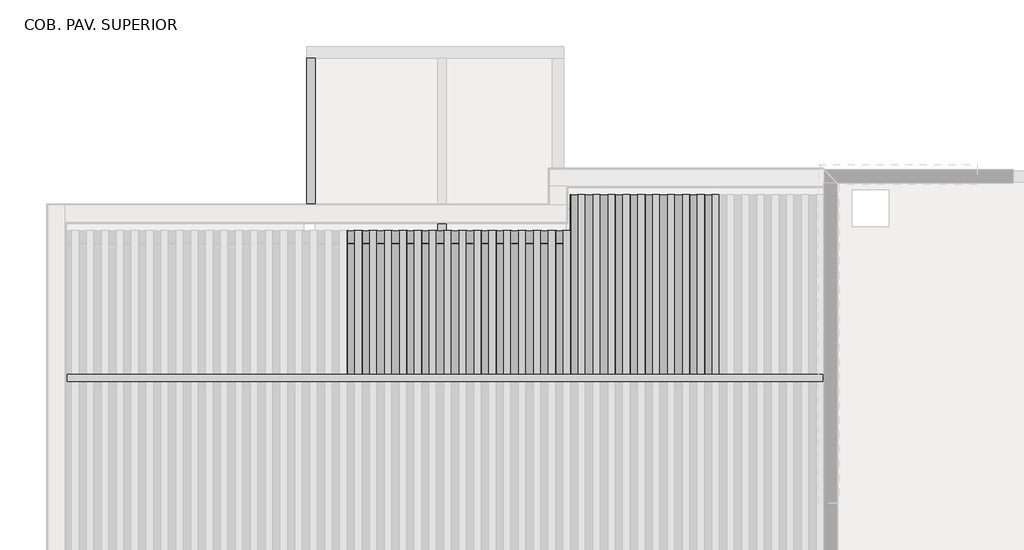
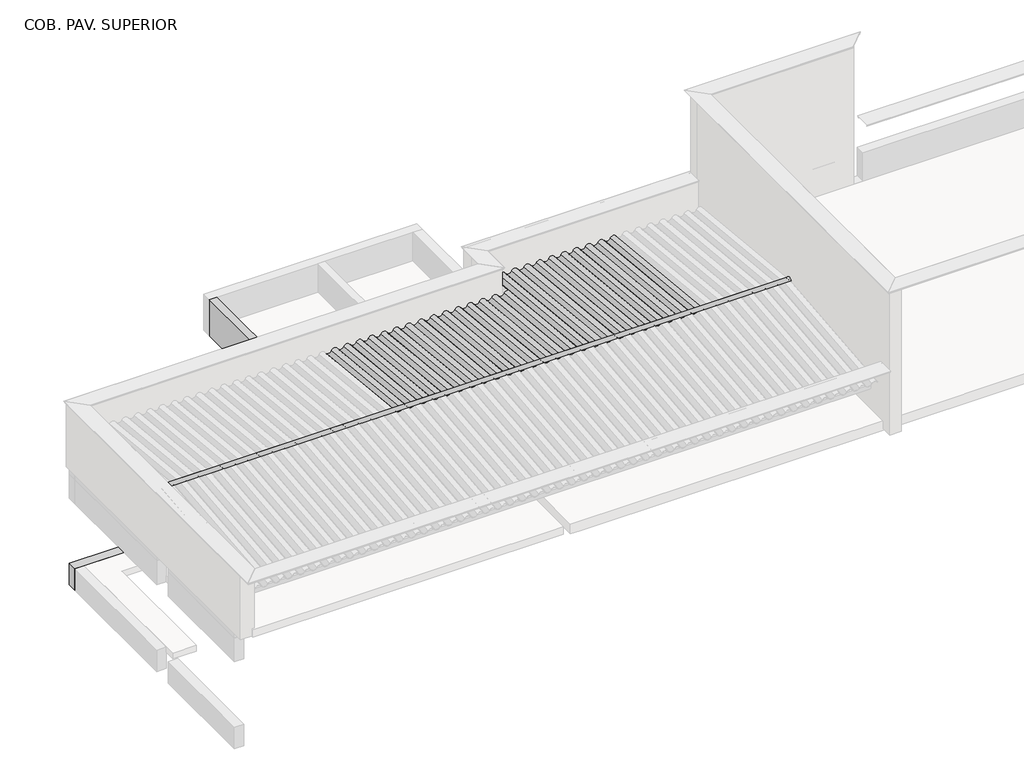
# One storey, part 4 of 7: 41 beams, 9 columns.
# Revit data of these elements (continued)
# Type "Madeira de lei : Berço 6x12cm"
#   A = 0.02 m²
#   Length [instance default] = 1.524 m
#   b = 0.06 m
#   d = 0.12 m
#   Structural Material [instance default] = none
#   Assembly Code = ""
# Type "Cumeeira Telha Ondulada : Fibrocimento"
#   Cost = 5
#   Length [instance default] = 1.524 m
#   b = 0.07 m
#   h = 0.16 m
#   Structural Material = .TELHA DE FIBROCIMENTO
#   Assembly Code = ""
# Type "TQS - Viga retangular : 14.0 x 76.0"
#   Length [instance default] = 1.524 m
#   b = 0.14 m
#   h = 0.76 m
#   Structural Material [instance default] = none
#   Assembly Code = ""
# Type "TQS - Viga retangular : 19.0 x 45.0"
#   Length [instance default] = 1.524 m
#   b = 0.19 m
#   h = 0.45 m
#   Structural Material [instance default] = none
#   Assembly Code = ""
# Type "TQS - Viga retangular : 19.0 x 96.0"
#   Length [instance default] = 1.524 m
#   b = 0.19 m
#   h = 0.96 m
#   Structural Material [instance default] = none
#   Assembly Code = ""
# Type "Telha Ondulada : Fibrocimento"
#   Description = "TELHA ONDULADA FIBROCIMENTO"
#   Cost = 5
#   Length [instance default] = 1.524 m
#   b = 0.07 m
#   h = 0.16 m
#   Structural Material = .TELHA DE FIBROCIMENTO
#   Assembly Code = ""
# Type "Madeira de lei : Viga Cumeeira 6x16cm"
#   A = 0.02 m²
#   Length [instance default] = 1.524 m
#   b = 0.06 m
#   d = 0.16 m
#   Structural Material [instance default] = none
#   Assembly Code = ""
# Type "Madeira de lei-Coluna : Pontalete 6X16cm"
#   A = 0.01952 m²
#   b = 0.06 m
#   d = 0.16 m
#   Structural Material [instance default] = none
#   Assembly Code = ""
# Elements 1, 2, 3, 4, 5, 6, 7, 8, 9 (IfcBeam, "Madeira de lei : Berço 6x12cm")
#   Comments = ""
#   Structural Material = .MADEIRAMENTO
#   Phase Created = CC_PE
#   Materials on its faces: ".MADEIRAMENTO"
# Element 10 (IfcBeam, "Cumeeira Telha Ondulada : Fibrocimento")
#   Comments = ""
#   Phase Created = CC_PE
#   Materials on its faces: ".TELHA DE FIBROCIMENTO"
# Element 11 (IfcBeam, "TQS - Viga retangular : 14.0 x 76.0")
#   Uso = "ESTRUTURA"
#   Titulo = "V415"
#   Chave = "-398"
#   Tipo Elemento = "Viga"
#   SHA1 = "2AA376B6A26CF9712D89C0E8D11BC49B460EBC49"
#   Revisão = ""
#   Tipo de carga = ""
#   Divisor de flexao = ""
#   Secao = ""
#   Configuracao = ""
#   Angulo (graus) = ""
#   Detalhamento = ""
#   Casos de vento manual = ""
#   Tipo = ""
#   Alcas = ""
#   Furos = ""
#   Pino = ""
#   Distribuicao = ""
#   Solidarizado = ""
#   Solidarizar na montagem = ""
#   Unir com o próximo = ""
#   Grupo pre moldado = ""
#   Verificado = ""
#   Concreto C = ""
#   Taxa de armadura (kgf/m³) = 0
#   Carga (tf/m²) = 0
#   Carga (tf/m) = 0
#   Carga (tf) = 0
#   Altura = 0.76 m
#   Rebaixo = -0.40 m
#   Largura = 0.14 m
#   Distancia a face = 0.00 m
#   Distancia ao eixo = 0.00 m
#   Altura gerber esquerda = 0.00 m
#   Largura gerber esquerda = 0.00 m
#   Altura gerber direita = 0.00 m
#   Largura gerber direita = 0.00 m
#   Resultado de Ensaios fck (MPa) = 0
#   Unique TQS ID = -398
#   Principal = yes
#   Structural Material = none
#   Phase Created = CC_PE
# Element 12 (IfcBeam, "TQS - Viga retangular : 14.0 x 76.0")
#   Uso = "ESTRUTURA"
#   Titulo = "V417"
#   Chave = "-400"
#   Tipo Elemento = "Viga"
#   SHA1 = "12908E79E151D5AD934E49BC800BD2D4B155789F"
#   Revisão = ""
#   Tipo de carga = ""
#   Divisor de flexao = ""
#   Secao = ""
#   Configuracao = ""
#   Angulo (graus) = ""
#   Detalhamento = ""
#   Casos de vento manual = ""
#   Tipo = ""
#   Alcas = ""
#   Furos = ""
#   Pino = ""
#   Distribuicao = ""
#   Solidarizado = ""
#   Solidarizar na montagem = ""
#   Unir com o próximo = ""
#   Grupo pre moldado = ""
#   Verificado = ""
#   Concreto C = ""
#   Taxa de armadura (kgf/m³) = 0
#   Carga (tf/m²) = 0
#   Carga (tf/m) = 0
#   Carga (tf) = 0
#   Altura = 0.76 m
#   Rebaixo = -0.40 m
#   Largura = 0.14 m
#   Distancia a face = 0.00 m
#   Distancia ao eixo = 0.00 m
#   Altura gerber esquerda = 0.00 m
#   Largura gerber esquerda = 0.00 m
#   Altura gerber direita = 0.00 m
#   Largura gerber direita = 0.00 m
#   Resultado de Ensaios fck (MPa) = 0
#   Unique TQS ID = -400
#   Principal = yes
#   Structural Material = none
#   Phase Created = CC_PE
# Element 13 (IfcBeam, "TQS - Viga retangular : 19.0 x 45.0")
#   Uso = "ESTRUTURA"
#   Titulo = "V406"
#   Chave = "-489"
#   Tipo Elemento = "Viga"
#   SHA1 = "B7AD3A1763948BDE1A611904C75AEF1C9438F7E4"
#   Revisão = ""
#   Tipo de carga = ""
#   Divisor de flexao = ""
#   Secao = ""
#   Configuracao = ""
#   Angulo (graus) = ""
#   Detalhamento = ""
#   Casos de vento manual = ""
#   Tipo = ""
#   Alcas = ""
#   Furos = ""
#   Pino = ""
#   Distribuicao = ""
#   Solidarizado = ""
#   Solidarizar na montagem = ""
#   Unir com o próximo = ""
#   Grupo pre moldado = ""
#   Verificado = ""
#   Concreto C = ""
#   Taxa de armadura (kgf/m³) = 0
#   Carga (tf/m²) = 0
#   Carga (tf/m) = 0
#   Carga (tf) = 0
#   Altura = 0.45 m
#   Rebaixo = 0.00 m
#   Largura = 0.19 m
#   Distancia a face = 0.00 m
#   Distancia ao eixo = 0.00 m
#   Altura gerber esquerda = 0.00 m
#   Largura gerber esquerda = 0.00 m
#   Altura gerber direita = 0.00 m
#   Largura gerber direita = 0.00 m
#   Resultado de Ensaios fck (MPa) = 0
#   Unique TQS ID = -489
#   Principal = yes
#   Structural Material = none
#   Phase Created = CC_PE
# Element 14 (IfcBeam, "TQS - Viga retangular : 19.0 x 96.0")
#   Uso = "ESTRUTURA"
#   Titulo = "V418"
#   Chave = "-411"
#   Tipo Elemento = "Viga"
#   SHA1 = "D9FA2317A6311B9903F22CD982B7CD8B04AEE9C1"
#   Revisão = ""
#   Tipo de carga = ""
#   Divisor de flexao = ""
#   Secao = ""
#   Configuracao = ""
#   Angulo (graus) = ""
#   Detalhamento = ""
#   Casos de vento manual = ""
#   Tipo = ""
#   Alcas = ""
#   Furos = ""
#   Pino = ""
#   Distribuicao = ""
#   Solidarizado = ""
#   Solidarizar na montagem = ""
#   Unir com o próximo = ""
#   Grupo pre moldado = ""
#   Verificado = ""
#   Concreto C = ""
#   Taxa de armadura (kgf/m³) = 0
#   Carga (tf/m²) = 0
#   Carga (tf/m) = 0
#   Carga (tf) = 0
#   Altura = 0.96 m
#   Rebaixo = -0.60 m
#   Largura = 0.19 m
#   Distancia a face = 0.00 m
#   Distancia ao eixo = 0.00 m
#   Altura gerber esquerda = 0.00 m
#   Largura gerber esquerda = 0.00 m
#   Altura gerber direita = 0.00 m
#   Largura gerber direita = 0.00 m
#   Resultado de Ensaios fck (MPa) = 0
#   Unique TQS ID = -411
#   Principal = yes
#   Structural Material = none
#   Phase Created = CC_PE
# Element 15 (IfcBeam, "TQS - Viga retangular : 19.0 x 96.0")
#   Uso = "ESTRUTURA"
#   Titulo = "V407"
#   Chave = "-511"
#   Tipo Elemento = "Viga"
#   SHA1 = "96EC062E150E290B67ABAE94CC465500946A7884"
#   Revisão = ""
#   Tipo de carga = ""
#   Divisor de flexao = ""
#   Secao = ""
#   Configuracao = ""
#   Angulo (graus) = ""
#   Detalhamento = ""
#   Casos de vento manual = ""
#   Tipo = ""
#   Alcas = ""
#   Furos = ""
#   Pino = ""
#   Distribuicao = ""
#   Solidarizado = ""
#   Solidarizar na montagem = ""
#   Unir com o próximo = ""
#   Grupo pre moldado = ""
#   Verificado = ""
#   Concreto C = ""
#   Taxa de armadura (kgf/m³) = 0
#   Carga (tf/m²) = 0
#   Carga (tf/m) = 0
#   Carga (tf) = 0
#   Altura = 0.96 m
#   Rebaixo = -0.60 m
#   Largura = 0.19 m
#   Distancia a face = 0.00 m
#   Distancia ao eixo = 0.00 m
#   Altura gerber esquerda = 0.00 m
#   Largura gerber esquerda = 0.00 m
#   Altura gerber direita = 0.00 m
#   Largura gerber direita = 0.00 m
#   Resultado de Ensaios fck (MPa) = 0
#   Unique TQS ID = -511
#   Principal = yes
#   Structural Material = none
#   Phase Created = CC_PE
# Elements 16, 17, 18, 19, 20, 21, 22, 23, 24, 25, 26, 27, 28, 29, 30, 31, 32, 33, 34, 35, 36, 37, 38, 39, 40 (IfcBeam, "Telha Ondulada : Fibrocimento")
#   Phase Created = CC_PE
#   Materials on its faces: ".TELHA DE FIBROCIMENTO"
# Element 41 (IfcBeam, "Madeira de lei : Viga Cumeeira 6x16cm")
#   Comments = ""
#   Structural Material = .MADEIRAMENTO
#   Phase Created = CC_PE
#   Materials on its faces: ".MADEIRAMENTO"
# Elements 42, 43, 44, 45, 46, 47, 48, 49, 50 (IfcColumn, "Madeira de lei-Coluna : Pontalete 6X16cm")
#   Comments = ""
#   Structural Material = .MADEIRAMENTO
#   Phase Created = CC_PE
#   Materials on its faces: ".MADEIRAMENTO"
# Materials
#   ".TELHA DE FIBROCIMENTO": class "CC_TELHADO", colour RGB 77 77 76, transparency 0, Description = "TELHA ONDULADA FIBROCIMENTO", Cost = 0
#   ".MADEIRAMENTO": class ".CC_MADEIRAS", colour RGB 212 179 113, transparency 0, Cost = 0
